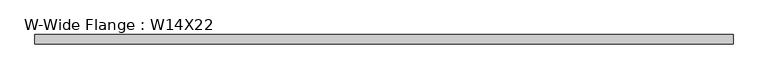
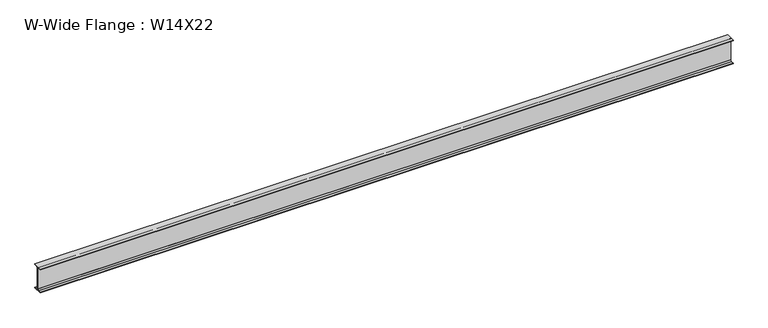
"""IFC4 building model written with IfcOpenShell, lengths in millimetres: beam geometry, W-Wide Flange : W14X22."""

from ifc_helpers import new_model, si_unit, point, frame, frame_2d, origin, place, context, project, spatial, polyline, circle_curve, trimmed, segment, composite_curve, outline, extrude, source, transform, mapped, element, save


def w_wide_flange_w14x22_9bef81b0(model_context):
    return source(origin(), model_context, "Body", "SweptSolid", [
        extrude(outline(composite_curve([segment(polyline([(63.5, -165.481), (63.5, -173.99), (-63.5, -173.99), (-63.5, -165.481), (-21.3995, -165.481)]), True, "CONTINUOUS"), segment(trimmed(circle_curve(frame_2d((-21.3995, -147.0025)), 18.4785), [point((-21.3995, -165.481))], [point((-2.921, -147.0025))], True, "CARTESIAN"), True, "CONTINUOUS"), segment(polyline([(-2.921, -147.0025), (-2.921, 147.0025)]), True, "CONTINUOUS"), segment(trimmed(circle_curve(frame_2d((-21.3995, 147.0025)), 18.4785), [point((-2.921, 147.0025))], [point((-21.3995, 165.481))], True, "CARTESIAN"), True, "CONTINUOUS"), segment(polyline([(-21.3995, 165.481), (-63.5, 165.481), (-63.5, 173.99), (63.5, 173.99), (63.5, 165.481), (21.3995, 165.481)]), True, "CONTINUOUS"), segment(trimmed(circle_curve(frame_2d((21.3995, 147.0025)), 18.4785), [point((21.3995, 165.481))], [point((2.921, 147.0025))], True, "CARTESIAN"), True, "CONTINUOUS"), segment(polyline([(2.921, 147.0025), (2.921, -147.0025)]), True, "CONTINUOUS"), segment(trimmed(circle_curve(frame_2d((21.3995, -147.0025)), 18.4785), [point((2.921, -147.0025))], [point((21.3995, -165.481))], True, "CARTESIAN"), True, "CONTINUOUS"), segment(polyline([(21.3995, -165.481), (63.5, -165.481)]), True, "CONTINUOUS")], self_intersect=False)), frame((-4799.838, 0.0, 0.0), z_axis=(1.0, 0.0, 0.0), x_axis=(0.0, 1.0, 0.0)), (0.0, 0.0, 1.0), 9594.088),
    ])


if __name__ == "__main__":
    model = new_model("IFC4")
    model_context = context("Model", 3, world=origin())
    ifc_project = project(units=[si_unit("LENGTHUNIT", "METRE", prefix="MILLI")], contexts=[model_context])
    site = spatial("IfcSite", under=ifc_project)
    building = spatial("IfcBuilding", under=site)
    placement = place(None, origin())
    w_wide_flange_w14x22_shape = w_wide_flange_w14x22_9bef81b0(model_context)
    element("IfcBeam", 1, ObjectType="W-Wide Flange : W14X22", at=placement, inside=building, context=model_context, shape_type="MappedRepresentation", body=[
        mapped(w_wide_flange_w14x22_shape, transform((0.0, 0.0, 0.0), x_axis=(1.0, 0.0, 0.0), y_axis=(0.0, 1.0, 0.0), z_axis=(0.0, 0.0, 1.0))),
    ])
    save(model, "model.ifc")

# Revit data of these elements
# Type "W-Wide Flange : W14X22"
#   Assembly Code = "B10"
#   W = 22
#   Length [instance default] = 1524 mm
#   bf = 127 mm
#   d = 347.98 mm
#   k = 26.988 mm
#   k2 = 18.479 mm
#   tf = 8.509 mm
#   tw = 5.842 mm
#   A = 0.00418709 m²
#   Structural Material [instance default] = Steel ASTM A992
# Element 1 (IfcBeam, "W-Wide Flange : W14X22")
#   Structural Material = Aluminum, Anodized Red
#   Materials on its faces: "Aluminum, Anodized Red"
# Materials
#   "Steel ASTM A992": class "Metal", colour RGB 128 0 0, transparency 0, Description = "Structural steel 50ksi", Cost = 0
#   "Aluminum, Anodized Red": class "Metal", colour RGB 120 120 120, transparency 0, Description = "Anodized aluminum, red", Cost = 0
